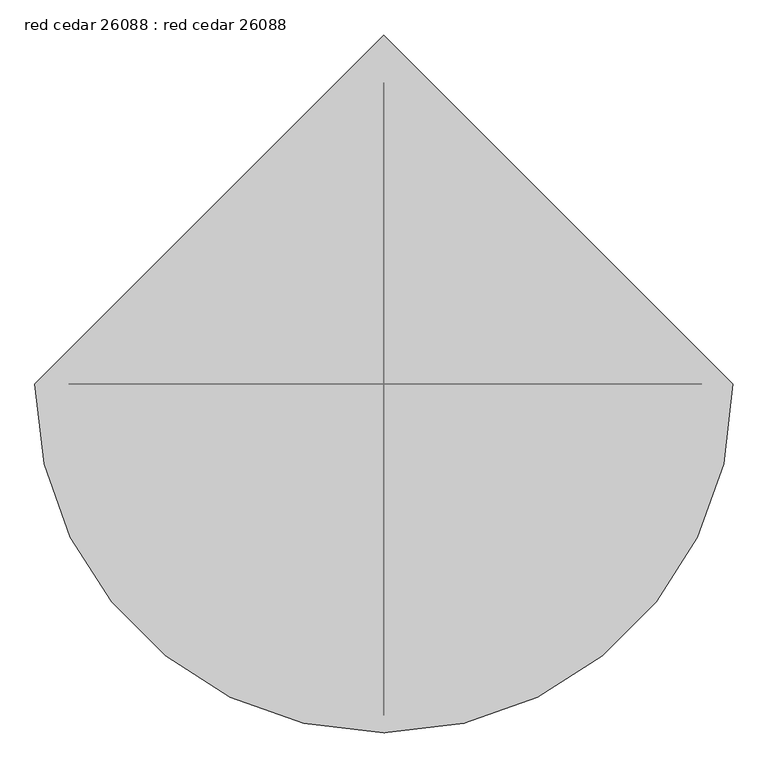
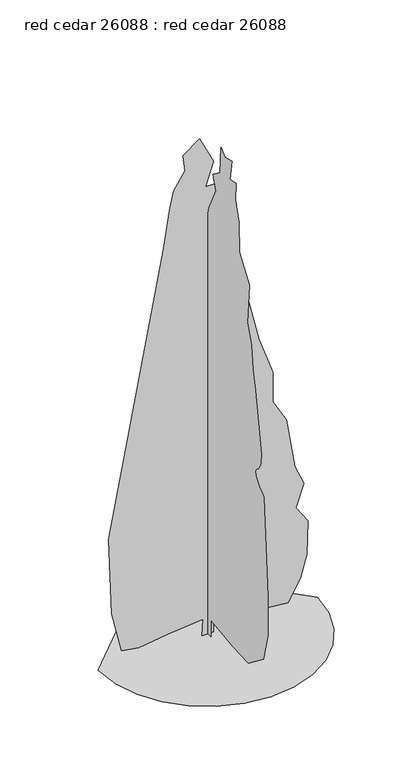
"""IFC4 building model written with IfcOpenShell, lengths in millimetres: proxy geometry, red cedar 26088 : red cedar 26088."""

from ifc_helpers import new_model, si_unit, origin, place, context, project, spatial, triangles, source, transform, mapped, element, save


def red_cedar_26088_red_cedar_26088_a2d53891(model_context):
    return source(origin(), model_context, "Body", "Tessellation", [
        triangles([(-33.5074115, 1.5e-06, 2.9e-06), (-28.3324185, -4.6e-06, 98.3225959), (-233.7142045, 5.5e-06, 79.3805562), (-399.8618937, 1.42e-05, 54.911224), (-499.2444177, 1.75e-05, 72.4481351), (-556.1683414, 5.5e-06, 315.6659792), (-571.6927935, -2.13e-05, 776.2313261), (-483.7199292, -5.29e-05, 1241.968087), (-256.0268143, -0.0001341, 2437.3627087), (-219.8026264, -0.0001489, 2659.8870621), (-199.1031631, -0.0001563, 2768.5481621), (-131.829753, -0.0001654, 2872.0531815), (-142.1794938, -0.0001705, 2965.1948799), (-49.0318863, -0.0001789, 3037.6610962), (33.7659849, -0.0001727, 2872.0531815), (-12.8077666, -0.0001623, 2732.3276985), (49.2907141, -0.000165, 2732.3276985), (295.6025418, -0.0001139, 1694.3850941), (375.3077239, -0.0001037, 1464.4872082), (375.3077239, -9.29e-05, 1283.3674496), (452.9300935, -8.83e-05, 1148.821229), (504.6800234, -7.23e-05, 843.5031647), (556.4274098, -6.75e-05, 724.4813599), (509.8539808, -5.74e-05, 589.9350666), (577.1283992, -5.42e-05, 486.4377502), (571.9518983, -4.2e-05, 284.6170386), (535.7289639, -3.24e-05, 150.0712722), (463.2805882, -2.18e-05, 25.8744608), (341.9448257, -1.73e-05, 40.1411272), (173.487521, -9.7e-06, 36.2241947), (33.7659849, -6.7e-06, 87.9728642), (33.7659849, -1.5e-06, 0.0), (1.3e-06, 29.3359728, 9.21e-05), (-6e-07, 39.6857044, 72.4483894), (6.3e-06, 118.2140961, 25.2313837), (8.9e-06, 262.2040898, 67.2733964), (9.3e-06, 231.1559123, 108.6723366), (1.77e-05, 422.6253662, 108.6723366), (2.22e-05, 505.4242367, 129.3717999), (2.81e-05, 520.9487251, 248.3938681), (3.32e-05, 546.8236719, 465.7393044), (3.52e-05, 510.5982305, 548.5356314), (4.13e-05, 515.7747313, 683.0819246), (4.36e-05, 479.5492536, 771.0548252), (4.75e-05, 464.0248014, 1003.9244047), (4.84e-05, 396.7529265, 1091.8973053), (5.8e-05, 303.6035432, 1531.7615902), (6.33e-05, 200.1064449, 1883.6530472), (6.59e-05, 127.6585687, 2142.3977188), (6.55e-05, 91.4343717, 2168.2701221), (7e-05, 60.3851723, 2302.8164154), (7.46e-05, -12.0630389, 2608.147197), (7.78e-05, -84.5113568, 2753.0287605), (7.72e-05, -53.4621528, 2835.8327179), (7.65e-05, -120.7355538, 2887.572583), (8.31e-05, -131.0852854, 3047.9988373), (7.97e-05, -172.484221, 3011.7783737), (7.74e-05, -239.7573677, 3027.2977753), (7.29e-05, -224.2328974, 2908.2733543), (7.09e-05, -281.1575659, 2918.6366753), (6.66e-05, -275.9810469, 2815.1316559), (6.56e-05, -312.2065247, 2701.2888954), (5.74e-05, -317.3804821, 2520.1615791), (5.24e-05, -419.0363411, 2380.6522167), (4.28e-05, -395.0028517, 2137.2211452), (3.63e-05, -436.4023232, 2028.5498714), (3.51e-05, -451.9267754, 1888.8270046), (2.89e-05, -477.8017585, 1774.9817734), (1.64e-05, -534.7256822, 1417.9137428), (1.56e-05, -534.5885176, 1400.1872086), (1.49e-05, -533.6385392, 1382.5493317), (1.43e-05, -531.0579191, 1365.0945831), (1.37e-05, -526.0338072, 1347.911475), (1.33e-05, -517.7508462, 1331.0889553), (1.32e-05, -505.3962951, 1314.7187336), (1.32e-05, -488.1522532, 1298.891938), (1.29e-05, -477.659507, 1280.543058), (1.17e-05, -482.7217343, 1258.2012531), (1e-05, -498.2538168, 1234.3506741), (8.1e-06, -519.178339, 1211.4779423), (6.3e-06, -540.4152695, 1192.0621943), (5e-06, -556.8820696, 1178.5925222), (1e-05, -563.4987805, 1173.5481354), (-1.16e-05, -601.9975571, 589.9350666), (-1.65e-05, -601.9975571, 351.891457), (-2.19e-05, -555.4241281, 181.1204671), (-2.03e-05, -405.3533463, 67.2733964), (-1.33e-05, -250.1068449, 72.4481351), (-2.5e-06, -32.7624306, 103.4973345), (-1.4e-06, -32.7624306, 8.84e-05), (-633.4046516, 0.0, 0.000118), (-616.6584354, -145.1342734, 0.0001086), (-568.9699219, -278.4169084, 9.86e-05), (-494.1517053, -396.0290245, 8.83e-05), (-396.0290245, -494.1517053, 7.82e-05), (-278.4169084, -568.9699219, 6.86e-05), (-145.1342734, -616.6584354, 5.99e-05), (2.78e-05, -633.4046516, 5.26e-05), (145.1342734, -616.6584354, 4.72e-05), (278.4169084, -568.9699219, 0.0001331), (396.0290245, -494.1517053, 0.0001324), (494.1542487, -396.0290245, 0.0001339), (568.9699219, -278.4169084, 4.88e-05), (616.6584354, -145.1342734, 5.47e-05), (633.4046516, 5.54e-05, 6.26e-05), (-8.33e-05, 633.4046516, 0.0001281)], [[13, 14, 15], [12, 13, 15], [12, 15, 16], [11, 12, 16], [32, 1, 2], [31, 32, 2], [10, 11, 16], [16, 17, 18], [10, 16, 18], [9, 10, 18], [8, 9, 18], [8, 18, 19], [8, 19, 20], [7, 8, 20], [7, 20, 21], [7, 21, 22], [6, 7, 22], [6, 22, 23], [6, 23, 24], [5, 6, 24], [4, 5, 24], [3, 4, 24], [2, 3, 24], [31, 2, 24], [30, 31, 24], [29, 30, 24], [29, 24, 25], [29, 25, 26], [29, 26, 27], [29, 27, 28], [55, 56, 57], [35, 36, 37], [57, 58, 59], [55, 57, 59], [59, 60, 61], [89, 90, 33], [89, 33, 34], [53, 54, 55], [55, 59, 61], [53, 55, 61], [53, 61, 62], [52, 53, 62], [52, 62, 63], [51, 52, 63], [51, 63, 64], [51, 64, 65], [50, 51, 65], [38, 39, 40], [34, 35, 37], [50, 65, 66], [50, 66, 67], [49, 50, 67], [48, 49, 67], [48, 67, 68], [47, 48, 68], [47, 68, 69], [46, 47, 69], [46, 69, 70], [46, 70, 71], [46, 71, 72], [46, 72, 73], [46, 73, 74], [46, 74, 75], [46, 75, 76], [46, 76, 77], [46, 77, 78], [46, 78, 79], [46, 79, 80], [37, 38, 40], [37, 40, 41], [37, 41, 42], [46, 80, 81], [82, 83, 84], [34, 37, 42], [89, 34, 42], [89, 42, 43], [89, 43, 44], [45, 46, 81], [44, 45, 81], [89, 44, 81], [88, 89, 81], [88, 81, 82], [88, 82, 84], [88, 84, 85], [88, 85, 86], [88, 86, 87], [105, 106, 91], [104, 105, 91], [104, 91, 92], [103, 104, 92], [103, 92, 93], [103, 93, 94], [102, 103, 94], [101, 102, 94], [101, 94, 95], [101, 95, 96], [101, 96, 97], [101, 97, 98], [101, 98, 99], [101, 99, 100]], closed=False),
    ])


if __name__ == "__main__":
    model = new_model("IFC4")
    model_context = context("Model", 3, world=origin())
    ifc_project = project(units=[si_unit("LENGTHUNIT", "METRE", prefix="MILLI")], contexts=[model_context])
    site = spatial("IfcSite", under=ifc_project)
    building = spatial("IfcBuilding", under=site)
    placement = place(None, origin())
    red_cedar_26088_red_cedar_26088_shape = red_cedar_26088_red_cedar_26088_a2d53891(model_context)
    element("IfcBuildingElementProxy", 1, Name="red cedar 26088 : red cedar 26088", ObjectType="red cedar 26088 : red cedar 26088", at=placement, inside=building, context=model_context, shape_type="MappedRepresentation", body=[
        mapped(red_cedar_26088_red_cedar_26088_shape, transform((0.0, 0.0, 0.0), x_axis=(1.0, 0.0, 0.0), y_axis=(0.0, 1.0, 0.0), z_axis=(0.0, 0.0, 1.0))),
    ])
    save(model, "model.ifc")

# Revit data of these elements
# Type "red cedar 26088 : red cedar 26088"
#   built-in parameter 1005195 = "RPC-16-FXGH-CPG0-PPQ3-C000-ST1L-LVER-AU"
#   Height = 0
